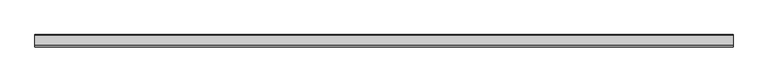
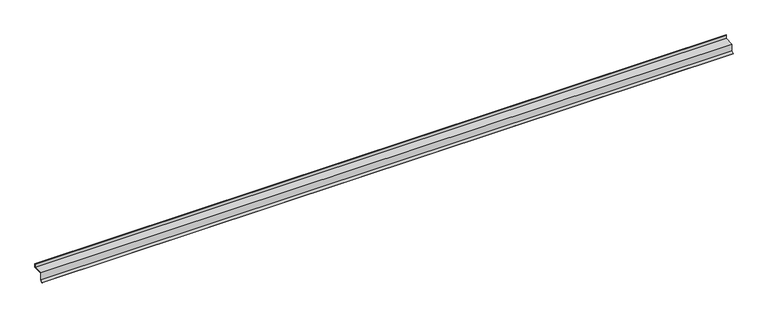
"""IFC4 building model written with IfcOpenShell, lengths in millimetres: proxy geometry, Generic Models 7:Generic Models 1:337419:Generic Models 1:337419 : Generic Models 7:Generic Models 1:337419:7 : Generic Models 7:Generic Models 1:337419:Generic Models 1:337419 : Generic Models 7:Generic Models 1:337419:301336."""

import ifcopenshell
import ifcopenshell.guid

model = None  # the IFC model being written
_history = None  # IfcOwnerHistory: only IFC2X3 demands one
_inside = {}  # id of a spatial element -> (the spatial element, [elements in it])
_under = {}  # id of a project, library or spatial element -> (it, [spatial elements below it])
_declared = {}  # id of a project -> (the project, [libraries it declares])
_typed = {}  # id of a type object -> (the type object, [elements of that type])
_made_of = {}  # id of a material, layer set ... -> (it, [elements and type objects made of it])


def new_model(schema):
    """Start an empty IFC model of exactly this schema.

    Asked for "IFC4X3", IfcOpenShell would pick the latest addendum, in which some entities
    have other attributes; the version numbers below select the first issue.
    IFC2X3 requires an IfcOwnerHistory on every rooted entity: one is made here for all.
    """
    global model, _history
    if schema == "IFC4X3":
        model = ifcopenshell.file(schema_version=(4, 3, 0, 0))
    else:
        model = ifcopenshell.file(schema=schema)
    _inside.clear()
    _under.clear()
    _declared.clear()
    _typed.clear()
    _made_of.clear()
    _history = None
    if model.schema == "IFC2X3":
        org = make("IfcOrganization", Name="unknown")
        user = make(
            "IfcPersonAndOrganization",
            ThePerson=make("IfcPerson", FamilyName="unknown"),
            TheOrganization=org,
        )
        app = make(
            "IfcApplication",
            ApplicationDeveloper=org,
            Version="unknown",
            ApplicationFullName="unknown",
            ApplicationIdentifier="unknown",
        )
        _history = make(
            "IfcOwnerHistory",
            OwningUser=user,
            OwningApplication=app,
            ChangeAction="ADDED",
            CreationDate=0,
        )
    return model


def make(cls, **values):
    """One entity of the class cls with the attributes given. An attribute that is None is left unset."""
    return model.create_entity(
        cls, **{name: value for name, value in values.items() if value is not None}
    )


def rooted(cls, **values):
    """An entity with a GlobalId (a new one), such as an element, a storey or a relation."""
    return make(cls, GlobalId=ifcopenshell.guid.new(), OwnerHistory=_history, **values)


def si_unit(unit_type, name, prefix=None):
    """IfcSIUnit, for example si_unit("LENGTHUNIT", "METRE", prefix="MILLI")."""
    return make("IfcSIUnit", UnitType=unit_type, Prefix=prefix, Name=name)


def assignment(units):
    """IfcUnitAssignment: the units of a project."""
    return None if units is None else make("IfcUnitAssignment", Units=units)


def point(xyz):
    """IfcCartesianPoint."""
    return None if xyz is None else make("IfcCartesianPoint", Coordinates=xyz)


def direction(xyz):
    """IfcDirection."""
    return None if xyz is None else make("IfcDirection", DirectionRatios=xyz)


def frame(location, z_axis=None, x_axis=None):
    """IfcAxis2Placement3D, a coordinate frame: its origin and axes. An axis left out is left unset."""
    return make(
        "IfcAxis2Placement3D",
        Location=point(location),
        Axis=direction(z_axis),
        RefDirection=direction(x_axis),
    )


def origin():
    """The frame at (0, 0, 0) with its axes left unset."""
    return frame((0.0, 0.0, 0.0))


def place(relative_to, where):
    """IfcLocalPlacement: puts the frame where relative to a parent placement (None: the world)."""
    return make(
        "IfcLocalPlacement", PlacementRelTo=relative_to, RelativePlacement=where
    )


def context(
    kind, dimensions, precision=None, world=None, true_north=None, identifier=None
):
    """IfcGeometricRepresentationContext, for example the 3D "Model" context."""
    return make(
        "IfcGeometricRepresentationContext",
        ContextIdentifier=identifier,
        ContextType=kind,
        CoordinateSpaceDimension=dimensions,
        Precision=precision,
        WorldCoordinateSystem=world,
        TrueNorth=true_north,
    )


def project(units=None, contexts=None):
    """IfcProject with its units and contexts."""
    return rooted(
        "IfcProject",
        Name="project",
        RepresentationContexts=contexts,
        UnitsInContext=assignment(units),
    )


def spatial(cls, under=None, at=None, **own):
    """A site, building, storey or space (cls), placed at a placement, below another one or the project."""
    s = rooted(cls, ObjectPlacement=at, **own)
    if under is not None:
        _under.setdefault(under.id(), (under, []))[1].append(s)
    return s


def polyline(points):
    """IfcPolyline through the points."""
    return make("IfcPolyline", Points=[point(p) for p in points])


def outline(outer, holes=None, kind="AREA"):
    """IfcArbitraryClosedProfileDef: a profile drawn as a closed curve; with holes, ...WithVoids."""
    if holes is None:
        return make("IfcArbitraryClosedProfileDef", ProfileType=kind, OuterCurve=outer)
    return make(
        "IfcArbitraryProfileDefWithVoids",
        ProfileType=kind,
        OuterCurve=outer,
        InnerCurves=holes,
    )


def extrude(swept, where, along, depth):
    """IfcExtrudedAreaSolid: the profile swept, set in the frame where, extruded along a direction by depth."""
    return make(
        "IfcExtrudedAreaSolid",
        SweptArea=swept,
        Position=where,
        ExtrudedDirection=direction(along),
        Depth=depth,
    )


def shape(context_of_items, identifier, shape_type, items):
    """IfcShapeRepresentation: the items that make up one representation, for example the "Body"."""
    return make(
        "IfcShapeRepresentation",
        ContextOfItems=context_of_items,
        RepresentationIdentifier=identifier,
        RepresentationType=shape_type,
        Items=items,
    )


def source(mapping_origin, context_of_items, identifier, shape_type, items):
    """IfcRepresentationMap: a shape defined once, which mapped items show again and again."""
    return make(
        "IfcRepresentationMap",
        MappingOrigin=mapping_origin,
        MappedRepresentation=shape(context_of_items, identifier, shape_type, items),
    )


def transform(
    local_origin,
    x_axis=None,
    y_axis=None,
    z_axis=None,
    scale=None,
    scale2=None,
    scale3=None,
    uniform=True,
):
    """IfcCartesianTransformationOperator3D, or its non-uniform kind. x_axis, y_axis, z_axis: its Axis1, 2, 3."""
    if uniform:
        return make(
            "IfcCartesianTransformationOperator3D",
            Axis1=direction(x_axis),
            Axis2=direction(y_axis),
            LocalOrigin=point(local_origin),
            Scale=scale,
            Axis3=direction(z_axis),
        )
    return make(
        "IfcCartesianTransformationOperator3DnonUniform",
        Axis1=direction(x_axis),
        Axis2=direction(y_axis),
        LocalOrigin=point(local_origin),
        Scale=scale,
        Axis3=direction(z_axis),
        Scale2=scale2,
        Scale3=scale3,
    )


def mapped(mapping_source, mapping_target):
    """IfcMappedItem: shows the shape of a source again, moved by a transform."""
    return make(
        "IfcMappedItem", MappingSource=mapping_source, MappingTarget=mapping_target
    )


def made_of(thing, what):
    """Note that an element or type object is made of a material, layer set ...; save() writes the relation."""
    if what is not None:
        _made_of.setdefault(what.id(), (what, []))[1].append(thing)
    return thing


def element(
    cls,
    number,
    at=None,
    inside=None,
    cuts=None,
    type_object=None,
    material=None,
    context=None,
    identifier="Body",
    shape_type=None,
    held_by="IfcProductDefinitionShape",
    body=None,
    shapes=None,
    **own,
):
    """One element of the class cls, such as IfcWall. Its Tag is "e" and its number.

    at: its placement. inside: the storey or other place that contains it. cuts: it is an
    opening in that element (IfcRelVoidsElement). A single representation is given by context,
    identifier, shape_type and body (its items); several are given by shapes. held_by: the class
    of the entity that holds the representations. save() writes the other relations.
    """
    e = rooted(cls, Tag="e%d" % number, ObjectPlacement=at, **own)
    if body is not None:
        shapes = [shape(context, identifier, shape_type, body)]
    if shapes is not None:
        e.Representation = make(held_by, Representations=shapes)
    if inside is not None:
        _inside.setdefault(inside.id(), (inside, []))[1].append(e)
    if cuts is not None:
        rooted(
            "IfcRelVoidsElement", RelatingBuildingElement=cuts, RelatedOpeningElement=e
        )
    if type_object is not None:
        _typed.setdefault(type_object.id(), (type_object, []))[1].append(e)
    return made_of(e, material)


def aggregate(whole, parts):
    """IfcRelAggregates: a whole, such as a stair, and the parts it consists of."""
    return rooted("IfcRelAggregates", RelatingObject=whole, RelatedObjects=parts)


def save(model, path):
    """Write the relations noted so far, then the file.

    IfcRelAggregates (storeys below a building ...), IfcRelContainedInSpatialStructure (elements
    in a storey), IfcRelDefinesByType, IfcRelAssociatesMaterial and IfcRelDeclares: one each for
    every whole, place, type object, material and project.
    """
    for whole, parts in _under.values():
        aggregate(whole, parts)
    for where, things in _inside.values():
        rooted(
            "IfcRelContainedInSpatialStructure",
            RelatedElements=things,
            RelatingStructure=where,
        )
    for kind, things in _typed.values():
        rooted("IfcRelDefinesByType", RelatedObjects=things, RelatingType=kind)
    for what, things in _made_of.values():
        rooted("IfcRelAssociatesMaterial", RelatedObjects=things, RelatingMaterial=what)
    for by, libraries in _declared.values():
        rooted("IfcRelDeclares", RelatingContext=by, RelatedDefinitions=libraries)
    model.write(path)


def generic_models_8dee9d38(model_context):
    return source(origin(), model_context, "Body", "SweptSolid", [
        extrude(outline(polyline([(-568181.0410514, 4904.3641712), (-568250.4941764, 4904.3641712), (-568250.4941764, 4855.1915591), (-568264.7782546, 4840.907481), (-568266.7426856, 4842.871912), (-568253.2723014, 4856.3422962), (-568253.2723014, 4907.1422962), (-568183.8191764, 4907.1422962), (-568183.8191764, 4931.7391922), (-568181.0410514, 4931.7391922), (-568181.0410514, 4904.3641712)])), frame((591306.0367242, 0.0, 0.0), z_axis=(1.0, 0.0, 0.0), x_axis=(0.0, 1.0, 0.0)), (0.0, 0.0, 1.0), 4876.8),
    ])


if __name__ == "__main__":
    model = new_model("IFC4")
    model_context = context("Model", 3, world=origin())
    ifc_project = project(units=[si_unit("LENGTHUNIT", "METRE", prefix="MILLI")], contexts=[model_context])
    site = spatial("IfcSite", under=ifc_project)
    building = spatial("IfcBuilding", under=site)
    placement = place(None, origin())
    generic_models_shape = generic_models_8dee9d38(model_context)
    element("IfcBuildingElementProxy", 1, Name="Generic Models 7:Generic Models 1:337419:Generic Models 1:337419 : Generic Models 7:Generic Models 1:337419:7 : Generic Models 7:Generic Models 1:337419:Generic Models 1:337419 : Generic Models 7:Generic Models 1:337419:301336", ObjectType="Generic Models 7:Generic Models 1:337419:Generic Models 1:337419 : Generic Models 7:Generic Models 1:337419:7 : Generic Models 7:Generic Models 1:337419:Generic Models 1:337419 : Generic Models 7:Generic Models 1:337419:301336", at=placement, inside=building, context=model_context, shape_type="MappedRepresentation", body=[
        mapped(generic_models_shape, transform((0.0, 0.0, 0.0), x_axis=(1.0, 0.0, 0.0), y_axis=(0.0, 1.0, 0.0), z_axis=(0.0, 0.0, 1.0))),
    ])
    save(model, "model.ifc")

# Revit data of these elements
# Type "Generic Models 7:Generic Models 1:337419:Generic Models 1:337419 : Generic Models 7:Generic Models 1:337419:7 : Generic Models 7:Generic Models 1:337419:Generic Models 1:337419 : Generic Models 7:Generic Models 1:337419:301336"
#   NameOverride = "Generic Models 7:Generic Models 1:337419:Generic Models 1:337419 : Generic Models 7:Generic Models 1:337419:301336"
#   ObjectTypeOverride = "Generic Models 1:337419 : Generic Models 7:Generic Models 1:337419"
#   Reference = "Generic Models 1"
#   Tag = "301336"
# Element 1 (IfcBuildingElementProxy, "Generic Models 7:Generic Models 1:337419:Generic Models 1:337419 : Generic Models 7:Generic Models 1:337419:7 : Generic Models 7:Generic Models 1:337419:Generic Models 1:337419 : Generic Models 7:Generic Models 1:337419:301336")
#   Materials on its faces: "BRAKE METAL FLASHING WITH BACK & END DAMS"
# Materials
#   "BRAKE METAL FLASHING WITH BACK & END DAMS": class "Unassigned", colour RGB 182 182 182, transparency 0, Cost = 0
